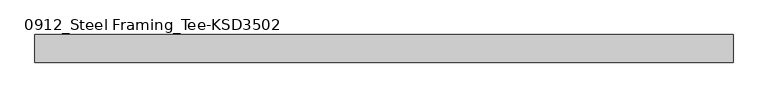
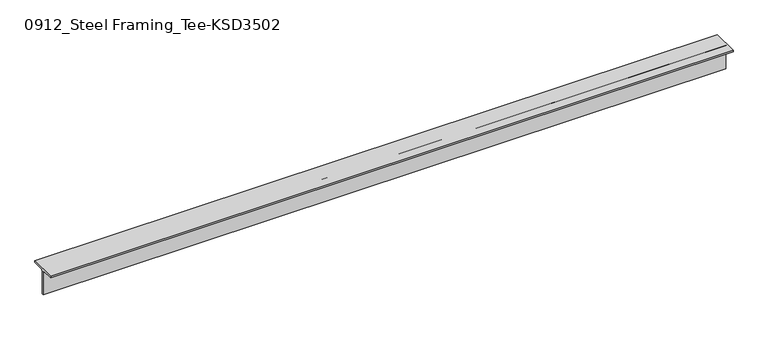
"""IFC4 building model written with IfcOpenShell, lengths in millimetres: member geometry, 0912_Steel Framing_Tee-KSD3502 : H_SB_ASB_CT-150x150x6.5x9."""

from ifc_helpers import new_model, si_unit, point, frame, frame_2d, origin, place, context, project, spatial, polyline, circle_curve, trimmed, segment, composite_curve, outline, extrude, source, transform, mapped, element, save


def member_0912_steel_framing_tee_ksd3502_ac3350f4(model_context):
    return source(origin(), model_context, "Body", "SweptSolid", [
        extrude(outline(composite_curve([segment(polyline([(-75.0, 75.0), (75.0, 75.0), (75.0, 66.0), (16.25, 66.0)]), True, "CONTINUOUS"), segment(trimmed(circle_curve(frame_2d((16.25, 53.0)), 13.0), [point((16.25, 66.0))], [point((3.25, 53.0))], True, "CARTESIAN"), True, "CONTINUOUS"), segment(polyline([(3.25, 53.0), (3.25, -75.0), (-3.25, -75.0), (-3.25, 53.0)]), True, "CONTINUOUS"), segment(trimmed(circle_curve(frame_2d((-16.25, 53.0)), 13.0), [point((-3.25, 53.0))], [point((-16.25, 66.0))], True, "CARTESIAN"), True, "CONTINUOUS"), segment(polyline([(-16.25, 66.0), (-75.0, 66.0), (-75.0, 75.0)]), True, "CONTINUOUS")], self_intersect=False)), frame((-1901.35, 0.0, 0.0), z_axis=(1.0, 0.0, 0.0), x_axis=(0.0, 1.0, 0.0)), (0.0, 0.0, 1.0), 3789.2),
    ])


if __name__ == "__main__":
    model = new_model("IFC4")
    model_context = context("Model", 3, world=origin())
    ifc_project = project(units=[si_unit("LENGTHUNIT", "METRE", prefix="MILLI")], contexts=[model_context])
    site = spatial("IfcSite", under=ifc_project)
    building = spatial("IfcBuilding", under=site)
    placement = place(None, origin())
    member_0912_steel_framing_tee_ksd3502_shape = member_0912_steel_framing_tee_ksd3502_ac3350f4(model_context)
    element("IfcMember", 1, ObjectType="0912_Steel Framing_Tee-KSD3502 : H_SB_ASB_CT-150x150x6.5x9", at=placement, inside=building, context=model_context, shape_type="MappedRepresentation", body=[
        mapped(member_0912_steel_framing_tee_ksd3502_shape, transform((0.0, 0.0, 0.0), x_axis=(1.0, 0.0, 0.0), y_axis=(0.0, 1.0, 0.0), z_axis=(0.0, 0.0, 1.0))),
    ])
    save(model, "model.ifc")

# Revit data of these elements
# Type "0912_Steel Framing_Tee-KSD3502 : H_SB_ASB_CT-150x150x6.5x9"
#   H_WM Code_1 = "S01AA003-00001 | Main Steel Structure Fabrication Work | Shelter/Building | Light Steel - Standard (30KG/M>Weight) | Material: (   )"
#   H_WM Code_2 = "S03AA029-00001 | Main Steel Structure Erection Work | Shelter/Building | Light Steel (30KG/M>Weight) | Material: (   )"
#   H_WM Code_3 = "S01AA010-00001 | Main Steel Structure Fabrication Work | Shelter/Building | Steel Painting/Coating | for Non-Fireproofed Steel Surface, Surface Preparation, Primer, Second & Final Coat | Material: (   )"
#   H_Q'ty Cal Type Tag = "SB-Q2"
#   Width = 15.0 cm
#   Web Thickness = 0.65 cm
#   Web Fillet = 1.3 cm
#   Section Area = 23.39 cm²
#   Perimeter = 0.60 m²/m
#   Nominal Weight = 18.40 kgf/m
#   Height = 15.0 cm
#   Flange Thickness = 0.9 cm
#   Centroid Vertical = 7.5 cm
#   Centroid Horizontal = 7.5 cm
#   Length [instance default] = 1.5000 m
#   Structural Material [instance default] = Steel, 45-345
#   Warping Constant = (empty or 0)
#   Torsional Moment of Inertia = 0
#   Section Name Key = ""
#   Plastic Modulus weak axis = 0
#   Plastic Modulus strong axis = 0
#   Moment of Inertia weak axis = 0
#   Moment of Inertia strong axis = 0
#   Elastic Modulus weak axis = 0
#   Elastic Modulus strong axis = 0
#   Bolt Spacing = 0
#   Assembly Code = ""
# Element 1 (IfcMember, "0912_Steel Framing_Tee-KSD3502 : H_SB_ASB_CT-150x150x6.5x9")
#   Structural Material = none
# Materials
#   "Steel, 45-345": class "Metal", colour RGB 189 187 185, transparency 0, Description = "Steel 345 MPa", Cost = 0
